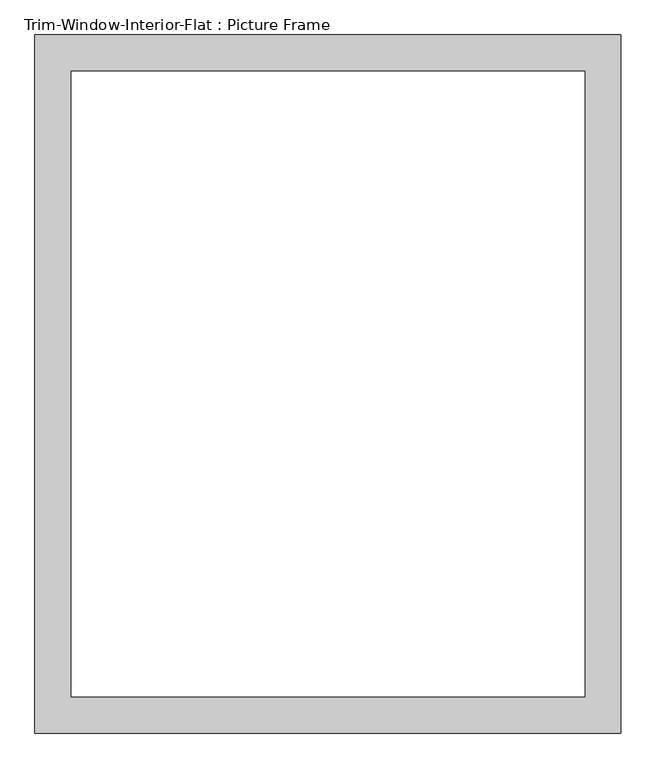
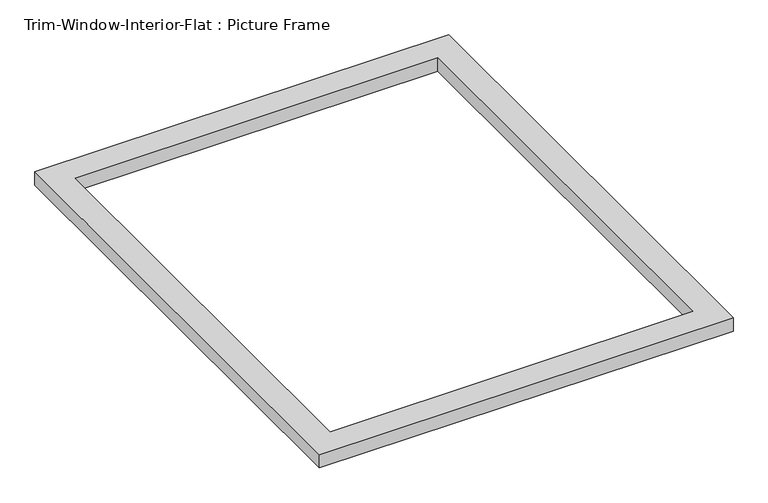
"""IFC4 building model written with IfcOpenShell, lengths in millimetres: proxy geometry, Trim-Window-Interior-Flat : Picture Frame."""

from ifc_helpers import new_model, si_unit, origin, origin_with_axes, place, context, project, spatial, polyline, outline, extrude, source, transform, mapped, element, save


def trim_window_interior_flat_picture_frame_996979b4(model_context):
    return source(origin(), model_context, "Body", "SweptSolid", [
        extrude(outline(polyline([(463.55, 44.45), (463.55, -1060.45), (-463.55, -1060.45), (-463.55, 44.45), (463.55, 44.45)]), holes=[polyline([(406.4, -12.7), (-406.4, -12.7), (-406.4, -1003.3), (406.4, -1003.3), (406.4, -12.7)])]), origin_with_axes(), (0.0, 0.0, 1.0), 31.75),
    ])


if __name__ == "__main__":
    model = new_model("IFC4")
    model_context = context("Model", 3, world=origin())
    ifc_project = project(units=[si_unit("LENGTHUNIT", "METRE", prefix="MILLI")], contexts=[model_context])
    site = spatial("IfcSite", under=ifc_project)
    building = spatial("IfcBuilding", under=site)
    placement = place(None, origin())
    trim_window_interior_flat_picture_frame_shape = trim_window_interior_flat_picture_frame_996979b4(model_context)
    element("IfcBuildingElementProxy", 1, Name="Trim-Window-Interior-Flat : Picture Frame", ObjectType="Trim-Window-Interior-Flat : Picture Frame", at=placement, inside=building, context=model_context, shape_type="MappedRepresentation", body=[
        mapped(trim_window_interior_flat_picture_frame_shape, transform((0.0, 0.0, 0.0), x_axis=(1.0, 0.0, 0.0), y_axis=(0.0, 1.0, 0.0), z_axis=(0.0, 0.0, 1.0))),
    ])
    save(model, "model.ifc")

# Revit data of these elements
# Type "Trim-Window-Interior-Flat : Picture Frame"
#   Trim Thickness_Picture Frame = 0' - 1 1/4"
#   Trim Width = 0' - 2 1/4"
#   Trim Thickness_with Sill = 0' - 0 3/4"
#   Sill Thickness = 0' - 1 1/4"
#   Opening Width [instance default] = 2' - 0"
#   Opening Height [instance default] = 3' - 0"
#   Default Elevation = 4' - 0"
#   Sill = no
#   Picture Frame = yes
#   Trim Material [instance default] = none
# Element 1 (IfcBuildingElementProxy, "Trim-Window-Interior-Flat : Picture Frame")
#   Opening Width = 2' - 9"
#   Opening Height = 3' - 4"
#   Trim Material = Wood - Stained
#   Materials on its faces: "Wood - Stained"
# Materials
#   "Wood - Stained": class "Wood", colour RGB 224 178 126, transparency 0, Cost = 0
